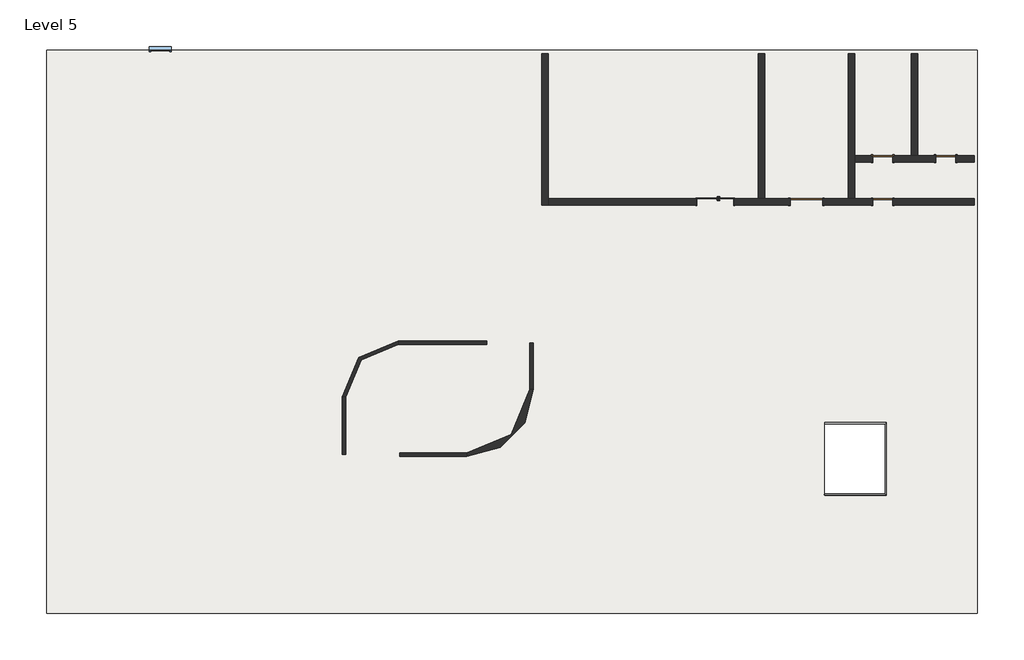
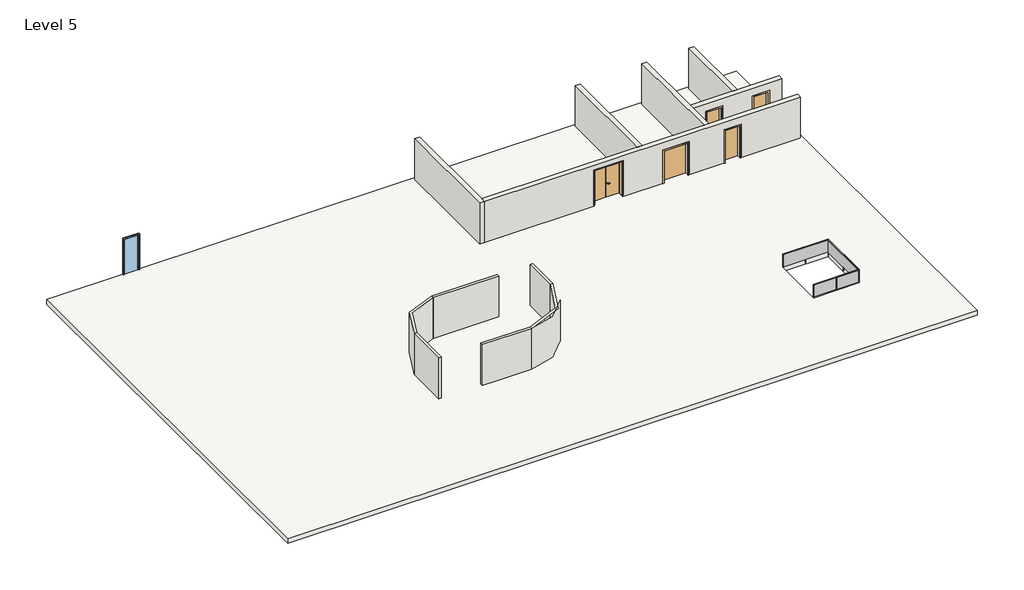
# One storey: 12 walls, 5 doors, 1 railing, 1 slab, 1 window.
"""IFC4 building model written with IfcOpenShell, lengths in millimetres."""

import ifcopenshell
import ifcopenshell.guid

model = None  # the IFC model being written
_history = None  # IfcOwnerHistory: only IFC2X3 demands one
_inside = {}  # id of a spatial element -> (the spatial element, [elements in it])
_under = {}  # id of a project, library or spatial element -> (it, [spatial elements below it])
_declared = {}  # id of a project -> (the project, [libraries it declares])
_typed = {}  # id of a type object -> (the type object, [elements of that type])
_made_of = {}  # id of a material, layer set ... -> (it, [elements and type objects made of it])


def new_model(schema):
    """Start an empty IFC model of exactly this schema.

    Asked for "IFC4X3", IfcOpenShell would pick the latest addendum, in which some entities
    have other attributes; the version numbers below select the first issue.
    IFC2X3 requires an IfcOwnerHistory on every rooted entity: one is made here for all.
    """
    global model, _history
    if schema == "IFC4X3":
        model = ifcopenshell.file(schema_version=(4, 3, 0, 0))
    else:
        model = ifcopenshell.file(schema=schema)
    _inside.clear()
    _under.clear()
    _declared.clear()
    _typed.clear()
    _made_of.clear()
    _history = None
    if model.schema == "IFC2X3":
        org = make("IfcOrganization", Name="unknown")
        user = make(
            "IfcPersonAndOrganization",
            ThePerson=make("IfcPerson", FamilyName="unknown"),
            TheOrganization=org,
        )
        app = make(
            "IfcApplication",
            ApplicationDeveloper=org,
            Version="unknown",
            ApplicationFullName="unknown",
            ApplicationIdentifier="unknown",
        )
        _history = make(
            "IfcOwnerHistory",
            OwningUser=user,
            OwningApplication=app,
            ChangeAction="ADDED",
            CreationDate=0,
        )
    return model


def make(cls, **values):
    """One entity of the class cls with the attributes given. An attribute that is None is left unset."""
    return model.create_entity(
        cls, **{name: value for name, value in values.items() if value is not None}
    )


def rooted(cls, **values):
    """An entity with a GlobalId (a new one), such as an element, a storey or a relation."""
    return make(cls, GlobalId=ifcopenshell.guid.new(), OwnerHistory=_history, **values)


def si_unit(unit_type, name, prefix=None):
    """IfcSIUnit, for example si_unit("LENGTHUNIT", "METRE", prefix="MILLI")."""
    return make("IfcSIUnit", UnitType=unit_type, Prefix=prefix, Name=name)


def assignment(units):
    """IfcUnitAssignment: the units of a project."""
    return None if units is None else make("IfcUnitAssignment", Units=units)


def point(xyz):
    """IfcCartesianPoint."""
    return None if xyz is None else make("IfcCartesianPoint", Coordinates=xyz)


def direction(xyz):
    """IfcDirection."""
    return None if xyz is None else make("IfcDirection", DirectionRatios=xyz)


def frame(location, z_axis=None, x_axis=None):
    """IfcAxis2Placement3D, a coordinate frame: its origin and axes. An axis left out is left unset."""
    return make(
        "IfcAxis2Placement3D",
        Location=point(location),
        Axis=direction(z_axis),
        RefDirection=direction(x_axis),
    )


def frame_2d(location, x_axis=None):
    """IfcAxis2Placement2D, a coordinate frame in the plane: its origin and x axis."""
    return make(
        "IfcAxis2Placement2D", Location=point(location), RefDirection=direction(x_axis)
    )


def origin():
    """The frame at (0, 0, 0) with its axes left unset."""
    return frame((0.0, 0.0, 0.0))


def origin_with_axes():
    """The frame at (0, 0, 0) with the z axis (0, 0, 1) and the x axis (1, 0, 0) written out."""
    return frame((0.0, 0.0, 0.0), z_axis=(0.0, 0.0, 1.0), x_axis=(1.0, 0.0, 0.0))


def place(relative_to, where):
    """IfcLocalPlacement: puts the frame where relative to a parent placement (None: the world)."""
    return make(
        "IfcLocalPlacement", PlacementRelTo=relative_to, RelativePlacement=where
    )


def context(
    kind, dimensions, precision=None, world=None, true_north=None, identifier=None
):
    """IfcGeometricRepresentationContext, for example the 3D "Model" context."""
    return make(
        "IfcGeometricRepresentationContext",
        ContextIdentifier=identifier,
        ContextType=kind,
        CoordinateSpaceDimension=dimensions,
        Precision=precision,
        WorldCoordinateSystem=world,
        TrueNorth=true_north,
    )


def project(units=None, contexts=None):
    """IfcProject with its units and contexts."""
    return rooted(
        "IfcProject",
        Name="project",
        RepresentationContexts=contexts,
        UnitsInContext=assignment(units),
    )


def spatial(cls, under=None, at=None, **own):
    """A site, building, storey or space (cls), placed at a placement, below another one or the project."""
    s = rooted(cls, ObjectPlacement=at, **own)
    if under is not None:
        _under.setdefault(under.id(), (under, []))[1].append(s)
    return s


def polyline(points):
    """IfcPolyline through the points."""
    return make("IfcPolyline", Points=[point(p) for p in points])


def circle_curve(where, radius):
    """IfcCircle in the frame where."""
    return make("IfcCircle", Position=where, Radius=radius)


def ellipse_curve(where, semi_axis1, semi_axis2):
    """IfcEllipse in the frame where."""
    return make(
        "IfcEllipse", Position=where, SemiAxis1=semi_axis1, SemiAxis2=semi_axis2
    )


def trimmed(basis, trim1, trim2, sense, master):
    """IfcTrimmedCurve: the piece of a basis curve between two trims."""
    return make(
        "IfcTrimmedCurve",
        BasisCurve=basis,
        Trim1=trim1,
        Trim2=trim2,
        SenseAgreement=sense,
        MasterRepresentation=master,
    )


def segment(curve, same_sense, transition):
    """IfcCompositeCurveSegment."""
    return make(
        "IfcCompositeCurveSegment",
        Transition=transition,
        SameSense=same_sense,
        ParentCurve=curve,
    )


def composite_curve(segments, self_intersect=None):
    """IfcCompositeCurve: segments joined end to end."""
    return make("IfcCompositeCurve", Segments=segments, SelfIntersect=self_intersect)


def outline(outer, holes=None, kind="AREA"):
    """IfcArbitraryClosedProfileDef: a profile drawn as a closed curve; with holes, ...WithVoids."""
    if holes is None:
        return make("IfcArbitraryClosedProfileDef", ProfileType=kind, OuterCurve=outer)
    return make(
        "IfcArbitraryProfileDefWithVoids",
        ProfileType=kind,
        OuterCurve=outer,
        InnerCurves=holes,
    )


def extrude(swept, where, along, depth):
    """IfcExtrudedAreaSolid: the profile swept, set in the frame where, extruded along a direction by depth."""
    return make(
        "IfcExtrudedAreaSolid",
        SweptArea=swept,
        Position=where,
        ExtrudedDirection=direction(along),
        Depth=depth,
    )


def faces_of(points, faces, orient=None, outer=None):
    """IfcFace entities. A face is a list of loops; a loop is a list of indices into points, from 0.

    orient and outer hold one flag for each loop. By default every Orientation is true, the
    first loop of a face is its IfcFaceOuterBound and the others are IfcFaceBound.
    """
    made = []
    for i, loops in enumerate(faces):
        bounds = []
        for j, loop in enumerate(loops):
            is_outer = j == 0 if outer is None else outer[i][j]
            bounds.append(
                make(
                    "IfcFaceOuterBound" if is_outer else "IfcFaceBound",
                    Bound=make("IfcPolyLoop", Polygon=[points[k] for k in loop]),
                    Orientation=True if orient is None else orient[i][j],
                )
            )
        made.append(make("IfcFace", Bounds=bounds))
    return made


def faceted_brep(points, faces, orient=None, outer=None, voids=None):
    """IfcFacetedBrep: a solid bounded by flat faces; with voids (closed shells), ...WithVoids."""
    shared = [point(p) for p in points]
    hull = make("IfcClosedShell", CfsFaces=faces_of(shared, faces, orient, outer))
    if voids is None:
        return make("IfcFacetedBrep", Outer=hull)
    return make(
        "IfcFacetedBrepWithVoids",
        Outer=hull,
        Voids=[
            make(cls, CfsFaces=faces_of(shared, fs, o, b)) for cls, fs, o, b in voids
        ],
    )


def shape(context_of_items, identifier, shape_type, items):
    """IfcShapeRepresentation: the items that make up one representation, for example the "Body"."""
    return make(
        "IfcShapeRepresentation",
        ContextOfItems=context_of_items,
        RepresentationIdentifier=identifier,
        RepresentationType=shape_type,
        Items=items,
    )


def source(mapping_origin, context_of_items, identifier, shape_type, items):
    """IfcRepresentationMap: a shape defined once, which mapped items show again and again."""
    return make(
        "IfcRepresentationMap",
        MappingOrigin=mapping_origin,
        MappedRepresentation=shape(context_of_items, identifier, shape_type, items),
    )


def transform(
    local_origin,
    x_axis=None,
    y_axis=None,
    z_axis=None,
    scale=None,
    scale2=None,
    scale3=None,
    uniform=True,
):
    """IfcCartesianTransformationOperator3D, or its non-uniform kind. x_axis, y_axis, z_axis: its Axis1, 2, 3."""
    if uniform:
        return make(
            "IfcCartesianTransformationOperator3D",
            Axis1=direction(x_axis),
            Axis2=direction(y_axis),
            LocalOrigin=point(local_origin),
            Scale=scale,
            Axis3=direction(z_axis),
        )
    return make(
        "IfcCartesianTransformationOperator3DnonUniform",
        Axis1=direction(x_axis),
        Axis2=direction(y_axis),
        LocalOrigin=point(local_origin),
        Scale=scale,
        Axis3=direction(z_axis),
        Scale2=scale2,
        Scale3=scale3,
    )


def mapped(mapping_source, mapping_target):
    """IfcMappedItem: shows the shape of a source again, moved by a transform."""
    return make(
        "IfcMappedItem", MappingSource=mapping_source, MappingTarget=mapping_target
    )


def made_of(thing, what):
    """Note that an element or type object is made of a material, layer set ...; save() writes the relation."""
    if what is not None:
        _made_of.setdefault(what.id(), (what, []))[1].append(thing)
    return thing


def element(
    cls,
    number,
    at=None,
    inside=None,
    cuts=None,
    type_object=None,
    material=None,
    context=None,
    identifier="Body",
    shape_type=None,
    held_by="IfcProductDefinitionShape",
    body=None,
    shapes=None,
    **own,
):
    """One element of the class cls, such as IfcWall. Its Tag is "e" and its number.

    at: its placement. inside: the storey or other place that contains it. cuts: it is an
    opening in that element (IfcRelVoidsElement). A single representation is given by context,
    identifier, shape_type and body (its items); several are given by shapes. held_by: the class
    of the entity that holds the representations. save() writes the other relations.
    """
    e = rooted(cls, Tag="e%d" % number, ObjectPlacement=at, **own)
    if body is not None:
        shapes = [shape(context, identifier, shape_type, body)]
    if shapes is not None:
        e.Representation = make(held_by, Representations=shapes)
    if inside is not None:
        _inside.setdefault(inside.id(), (inside, []))[1].append(e)
    if cuts is not None:
        rooted(
            "IfcRelVoidsElement", RelatingBuildingElement=cuts, RelatedOpeningElement=e
        )
    if type_object is not None:
        _typed.setdefault(type_object.id(), (type_object, []))[1].append(e)
    return made_of(e, material)


def aggregate(whole, parts):
    """IfcRelAggregates: a whole, such as a stair, and the parts it consists of."""
    return rooted("IfcRelAggregates", RelatingObject=whole, RelatedObjects=parts)


def save(model, path):
    """Write the relations noted so far, then the file.

    IfcRelAggregates (storeys below a building ...), IfcRelContainedInSpatialStructure (elements
    in a storey), IfcRelDefinesByType, IfcRelAssociatesMaterial and IfcRelDeclares: one each for
    every whole, place, type object, material and project.
    """
    for whole, parts in _under.values():
        aggregate(whole, parts)
    for where, things in _inside.values():
        rooted(
            "IfcRelContainedInSpatialStructure",
            RelatedElements=things,
            RelatingStructure=where,
        )
    for kind, things in _typed.values():
        rooted("IfcRelDefinesByType", RelatedObjects=things, RelatingType=kind)
    for what, things in _made_of.values():
        rooted("IfcRelAssociatesMaterial", RelatedObjects=things, RelatingMaterial=what)
    for by, libraries in _declared.values():
        rooted("IfcRelDeclares", RelatingContext=by, RelatedDefinitions=libraries)
    model.write(path)


def plane_surface(at):
    """IfcPlane: the flat surface through the origin of the frame at, square to its z axis."""
    return make("IfcPlane", Position=at)


def cylinder_surface(at, radius):
    """IfcCylindricalSurface: all points at the distance radius from the z axis of the frame at."""
    return make("IfcCylindricalSurface", Position=at, Radius=radius)


def advanced_brep(points, edges, surfaces, faces):
    """IfcAdvancedBrep: a solid bounded by faces that lie on surfaces and meet in shared edges.

    An edge is (start, end): straight between two places in points (the first is 0);
    or (start, end, curve); or (start, end, curve, False) where it runs against its curve.
    A face is (place in surfaces, loops), or (place, loops, False) where it looks against
    its surface's normal. A loop lists edges by number (the first is 1), with a minus sign
    where the edge is run from its end to its start. The first loop is the outer one.
    """
    corners = [point(p) for p in points]
    vertices = [make("IfcVertexPoint", VertexGeometry=c) for c in corners]
    made = []
    for start, end, *more in edges:
        made.append(
            make(
                "IfcEdgeCurve",
                EdgeStart=vertices[start],
                EdgeEnd=vertices[end],
                EdgeGeometry=more[0] if more else make("IfcPolyline", Points=[corners[start], corners[end]]),
                SameSense=more[1] if len(more) > 1 else True,
            )
        )
    hull = []
    for where, loops, *sense in faces:
        bounds = []
        for j, loop in enumerate(loops):
            ring = [make("IfcOrientedEdge", EdgeElement=made[abs(k) - 1], Orientation=k > 0) for k in loop]
            bounds.append(
                make(
                    "IfcFaceOuterBound" if j == 0 else "IfcFaceBound",
                    Bound=make("IfcEdgeLoop", EdgeList=ring),
                    Orientation=True,
                )
            )
        hull.append(make("IfcAdvancedFace", Bounds=bounds, FaceSurface=surfaces[where], SameSense=sense[0] if sense else True))
    return make("IfcAdvancedBrep", Outer=make("IfcClosedShell", CfsFaces=hull))


def door_double_flush_variable_door_double_flush_variable_ac6c3b87(model_context):
    return source(origin(), model_context, "Body", "SolidModel", [
        advanced_brep(
        [(90.0, 139.4346141, 1000.0), (110.0, 139.4346141, 1000.0), (90.0, 69.4346141, 1000.0), (110.0, 89.4346141, 1000.0), (220.0, 69.4346141, 1000.0), (220.0, 89.4346141, 1000.0)],
        [
            (0, 1, circle_curve(frame((100.0, 139.4346141, 1000.0), z_axis=(0.0, 1.0, 0.0), x_axis=(1.0, 0.0, 0.0)), 10.0)),
            (1, 0, circle_curve(frame((100.0, 139.4346141, 1000.0), z_axis=(0.0, 1.0, 0.0), x_axis=(1.0, 0.0, 0.0)), 10.0)),
            (0, 2),
            (2, 3, ellipse_curve(frame((100.0, 79.4346141, 1000.0), z_axis=(-0.7071067811865385, 0.7071067811865565, 0.0), x_axis=(0.7071067811865563, 0.7071067811865386, 0.0)), 14.1421356, 10.0)),
            (3, 1),
            (3, 2, ellipse_curve(frame((100.0, 79.4346141, 1000.0), z_axis=(-0.7071067811865385, 0.7071067811865565, 0.0), x_axis=(0.7071067811865563, 0.7071067811865386, 0.0)), 14.1421356, 10.0)),
            (4, 5, circle_curve(frame((220.0, 79.4346141, 1000.0), z_axis=(1.0, 0.0, 0.0), x_axis=(0.0, 1.0, 0.0)), 10.0)),
            (5, 4, circle_curve(frame((220.0, 79.4346141, 1000.0), z_axis=(1.0, 0.0, 0.0), x_axis=(0.0, 1.0, 0.0)), 10.0)),
            (2, 4),
            (5, 3),
        ],
        [
            plane_surface(frame((100.0, 139.4346141, -287.7526403), z_axis=(0.0, 1.0, 0.0), x_axis=(0.0, 0.0, 1.0))),
            cylinder_surface(frame((100.0, 139.4346141, 1000.0), z_axis=(0.0, 1.0, 0.0), x_axis=(1.0, 0.0, 0.0)), 10.0),
            plane_surface(frame((220.0, 79.4346141, -287.7526403), z_axis=(1.0, 0.0, 0.0), x_axis=(0.0, 0.0, 1.0))),
            cylinder_surface(frame((100.0, 79.4346141, 1000.0), z_axis=(-1.0, 0.0, 0.0), x_axis=(0.0, 1.0, 0.0)), 10.0),
        ],
        [
            (0, [[1, 2]]),
            (1, [[-1, 3, 4, 5]]),
            (1, [[-2, -5, 6, -3]]),
            (2, [[7, 8]]),
            (3, [[-4, 9, -8, 10]]),
            (3, [[-6, -10, -7, -9]]),
        ],
    ),
        advanced_brep(
        [(110.0, 199.4346141, 1000.0), (90.0, 199.4346141, 1000.0), (110.0, 229.4346141, 1000.0), (90.0, 249.4346141, 1000.0), (220.0, 229.4346141, 1000.0), (220.0, 249.4346141, 1000.0)],
        [
            (0, 1, circle_curve(frame((100.0, 199.4346141, 1000.0), z_axis=(0.0, -1.0, 0.0), x_axis=(-1.0, 0.0, 0.0)), 10.0)),
            (1, 0, circle_curve(frame((100.0, 199.4346141, 1000.0), z_axis=(0.0, -1.0, 0.0), x_axis=(-1.0, 0.0, 0.0)), 10.0)),
            (0, 2),
            (2, 3, ellipse_curve(frame((100.0, 239.4346141, 1000.0), z_axis=(-0.7071067811865475, -0.7071067811865475, 0.0), x_axis=(0.7071067811865474, -0.7071067811865476, 0.0)), 14.1421356, 10.0)),
            (3, 1),
            (3, 2, ellipse_curve(frame((100.0, 239.4346141, 1000.0), z_axis=(-0.7071067811865475, -0.7071067811865475, 0.0), x_axis=(0.7071067811865474, -0.7071067811865476, 0.0)), 14.1421356, 10.0)),
            (4, 5, circle_curve(frame((220.0, 239.4346141, 1000.0), z_axis=(1.0, 0.0, 0.0), x_axis=(0.0, 1.0, 0.0)), 10.0)),
            (5, 4, circle_curve(frame((220.0, 239.4346141, 1000.0), z_axis=(1.0, 0.0, 0.0), x_axis=(0.0, 1.0, 0.0)), 10.0)),
            (2, 4),
            (5, 3),
        ],
        [
            plane_surface(frame((100.0, 199.4346141, -287.7526403), z_axis=(0.0, -1.0, 0.0), x_axis=(0.0, 0.0, 1.0))),
            cylinder_surface(frame((100.0, 199.4346141, 1000.0), z_axis=(0.0, -1.0, 0.0), x_axis=(-1.0, 0.0, 0.0)), 10.0),
            plane_surface(frame((220.0, 239.4346141, -287.7526403), z_axis=(1.0, 0.0, 0.0), x_axis=(0.0, 0.0, 1.0))),
            cylinder_surface(frame((100.0, 239.4346141, 1000.0), z_axis=(-1.0, 0.0, 0.0), x_axis=(0.0, 1.0, 0.0)), 10.0),
        ],
        [
            (0, [[1, 2]]),
            (1, [[-1, 3, 4, 5]]),
            (1, [[-2, -5, 6, -3]]),
            (2, [[7, 8]]),
            (3, [[-4, 9, -8, 10]]),
            (3, [[-6, -10, -7, -9]]),
        ],
    ),
        extrude(outline(composite_curve([segment(trimmed(circle_curve(frame_2d((1000.0, 100.0)), 20.0), [point((1000.0, 80.0))], [point((1000.0, 120.0))], False, "CARTESIAN"), True, "CONTINUOUS"), segment(trimmed(circle_curve(frame_2d((1000.0, 100.0)), 20.0), [point((1000.0, 120.0))], [point((1000.0, 80.0))], False, "CARTESIAN"), True, "CONTINUOUS")], self_intersect=False)), frame((0.0, 129.4346141, 0.0), z_axis=(0.0, 1.0, 0.0), x_axis=(0.0, 0.0, 1.0)), (0.0, 0.0, 1.0), 10.0),
        extrude(outline(composite_curve([segment(trimmed(circle_curve(frame_2d((1000.0, 100.0)), 20.0), [point((1000.0, 80.0))], [point((1000.0, 120.0))], False, "CARTESIAN"), True, "CONTINUOUS"), segment(trimmed(circle_curve(frame_2d((1000.0, 100.0)), 20.0), [point((1000.0, 120.0))], [point((1000.0, 80.0))], False, "CARTESIAN"), True, "CONTINUOUS")], self_intersect=False)), frame((0.0, 189.4346141, 0.0), z_axis=(0.0, 1.0, 0.0), x_axis=(0.0, 0.0, 1.0)), (0.0, 0.0, 1.0), 10.0),
        extrude(outline(polyline([(0.0, 164.4346141), (-871.25, 164.4346141), (-871.25, 189.4346141), (0.0, 189.4346141), (0.0, 164.4346141)])), frame((0.0, 0.0, 100.0), z_axis=(0.0, 0.0, 1.0), x_axis=(1.0, 0.0, 0.0)), (0.0, 0.0, 1.0), 2250.0),
        extrude(outline(polyline([(871.25, 164.4346141), (0.0, 164.4346141), (0.0, 189.4346141), (871.25, 189.4346141), (871.25, 164.4346141)])), frame((0.0, 0.0, 100.0), z_axis=(0.0, 0.0, 1.0), x_axis=(1.0, 0.0, 0.0)), (0.0, 0.0, 1.0), 2250.0),
        faceted_brep([(905.75, -150.5653859, 100.0), (856.25, -150.5653859, 100.0), (856.25, 164.4346141, 100.0), (871.25, 164.4346141, 100.0), (871.25, 189.4346141, 100.0), (905.75, 189.4346141, 100.0), (905.75, 164.4346141, 100.0), (900.75, 164.4346141, 100.0), (900.75, 184.4346141, 100.0), (876.25, 184.4346141, 100.0), (876.25, 159.4346141, 100.0), (861.25, 159.4346141, 100.0), (861.25, -145.5653859, 100.0), (900.75, -145.5653859, 100.0), (900.75, -135.5653859, 100.0), (905.75, -135.5653859, 100.0), (905.75, -150.5653859, 2384.5), (-905.75, -150.5653859, 2384.5), (-905.75, -150.5653859, 100.0), (-856.25, -150.5653859, 100.0), (-856.25, -150.5653859, 2335.0), (856.25, -150.5653859, 2335.0), (856.25, 164.4346141, 2335.0), (-856.25, 164.4346141, 2335.0), (-856.25, 164.4346141, 100.0), (-871.25, 164.4346141, 100.0), (-871.25, 164.4346141, 2350.0), (871.25, 164.4346141, 2350.0), (871.25, 189.4346141, 2350.0), (-871.25, 189.4346141, 2350.0), (-871.25, 189.4346141, 100.0), (-905.75, 189.4346141, 100.0), (-905.75, 189.4346141, 2384.5), (905.75, 189.4346141, 2384.5), (905.75, 164.4346141, 2384.5), (-905.75, 164.4346141, 2384.5), (-905.75, 164.4346141, 100.0), (-900.75, 164.4346141, 100.0), (-900.75, 164.4346141, 2379.5), (900.75, 164.4346141, 2379.5), (900.75, 184.4346141, 2379.5), (-900.75, 184.4346141, 2379.5), (-900.75, 184.4346141, 100.0), (-876.25, 184.4346141, 100.0), (-876.25, 184.4346141, 2355.0), (876.25, 184.4346141, 2355.0), (876.25, 159.4346141, 2355.0), (-876.25, 159.4346141, 2355.0), (-876.25, 159.4346141, 100.0), (-861.25, 159.4346141, 100.0), (-861.25, 159.4346141, 2340.0), (861.25, 159.4346141, 2340.0), (861.25, -145.5653859, 2340.0), (-861.25, -145.5653859, 2340.0), (-861.25, -145.5653859, 100.0), (-900.75, -145.5653859, 100.0), (-900.75, -145.5653859, 2379.5), (900.75, -145.5653859, 2379.5), (900.75, -135.5653859, 2379.5), (-900.75, -135.5653859, 2379.5), (-900.75, -135.5653859, 100.0), (-905.75, -135.5653859, 100.0), (-905.75, -135.5653859, 2384.5), (905.75, -135.5653859, 2384.5)], [[[0, 1, 2, 3, 4, 5, 6, 7, 8, 9, 10, 11, 12, 13, 14, 15]], [[1, 0, 16, 17, 18, 19, 20, 21]], [[2, 1, 21, 22]], [[3, 2, 22, 23, 24, 25, 26, 27]], [[4, 3, 27, 28]], [[5, 4, 28, 29, 30, 31, 32, 33]], [[6, 5, 33, 34]], [[7, 6, 34, 35, 36, 37, 38, 39]], [[8, 7, 39, 40]], [[9, 8, 40, 41, 42, 43, 44, 45]], [[10, 9, 45, 46]], [[11, 10, 46, 47, 48, 49, 50, 51]], [[12, 11, 51, 52]], [[13, 12, 52, 53, 54, 55, 56, 57]], [[14, 13, 57, 58]], [[15, 14, 58, 59, 60, 61, 62, 63]], [[0, 15, 63, 16]], [[17, 62, 61, 18]], [[18, 61, 60, 55, 54, 49, 48, 43, 42, 37, 36, 31, 30, 25, 24, 19]], [[23, 20, 19, 24]], [[29, 26, 25, 30]], [[35, 32, 31, 36]], [[41, 38, 37, 42]], [[47, 44, 43, 48]], [[53, 50, 49, 54]], [[59, 56, 55, 60]], [[22, 21, 20, 23]], [[28, 27, 26, 29]], [[34, 33, 32, 35]], [[40, 39, 38, 41]], [[46, 45, 44, 47]], [[52, 51, 50, 53]], [[58, 57, 56, 59]], [[16, 63, 62, 17]]]),
    ])


def m_single_flush_0915_x_2134mm_1c84716f(model_context):
    return source(origin(), model_context, "Body", "SweptSolid", [
        extrude(outline(polyline([(2210.0, -533.5), (0.0, -533.5), (0.0, -457.5), (2134.0, -457.5), (2134.0, 457.5), (0.0, 457.5), (0.0, 533.5), (2210.0, 533.5), (2210.0, -533.5)])), frame((0.0, -175.0, 0.0), z_axis=(0.0, 1.0, 0.0), x_axis=(0.0, 0.0, 1.0)), (0.0, 0.0, 1.0), 25.0),
        extrude(outline(polyline([(2210.0, 533.5), (2210.0, -533.5), (0.0, -533.5), (0.0, -457.5), (2134.0, -457.5), (2134.0, 457.5), (0.0, 457.5), (0.0, 533.5), (2210.0, 533.5)])), frame((0.0, 150.0, 0.0), z_axis=(0.0, 1.0, 0.0), x_axis=(0.0, 0.0, 1.0)), (0.0, 0.0, 1.0), 25.0),
        extrude(outline(polyline([(457.5, -99.0), (457.5, -150.0), (-457.5, -150.0), (-457.5, -99.0), (457.5, -99.0)])), origin_with_axes(), (0.0, 0.0, 1.0), 2134.0),
    ])


def m_single_flush_1500_x_2134mm_2_edebd810(model_context):
    return source(origin(), model_context, "Body", "SweptSolid", [
        extrude(outline(polyline([(2210.0, -826.0), (0.0, -826.0), (0.0, -750.0), (2134.0, -750.0), (2134.0, 750.0), (0.0, 750.0), (0.0, 826.0), (2210.0, 826.0), (2210.0, -826.0)])), frame((0.0, -175.0, 0.0), z_axis=(0.0, 1.0, 0.0), x_axis=(0.0, 0.0, 1.0)), (0.0, 0.0, 1.0), 25.0),
        extrude(outline(polyline([(2210.0, 826.0), (2210.0, -826.0), (0.0, -826.0), (0.0, -750.0), (2134.0, -750.0), (2134.0, 750.0), (0.0, 750.0), (0.0, 826.0), (2210.0, 826.0)])), frame((0.0, 150.0, 0.0), z_axis=(0.0, 1.0, 0.0), x_axis=(0.0, 0.0, 1.0)), (0.0, 0.0, 1.0), 25.0),
        extrude(outline(polyline([(750.0, -99.0), (750.0, -150.0), (-750.0, -150.0), (-750.0, -99.0), (750.0, -99.0)])), origin_with_axes(), (0.0, 0.0, 1.0), 2134.0),
    ])


def glas_mpk_ffa405cb(model_context):
    return source(origin(), model_context, "Body", "SolidModel", [
        faceted_brep([(29194.1667192, -1196.642277, 12843.2628643), (29194.1667192, -1246.642277, 12843.2628643), (29194.1667192, -1246.642277, 12856.7371357), (29194.1667192, -1196.642277, 12856.7371357), (32034.1667192, -1196.642277, 12843.2628643), (31984.1667192, -1246.642277, 12843.2628643), (31984.1667192, -1246.642277, 12856.7371357), (32034.1667192, -1196.642277, 12856.7371357), (32034.1667192, -4537.3716232, 12843.2628643), (31984.1667192, -4487.3716232, 12843.2628643), (31984.1667192, -4487.3716232, 12856.7371357), (32034.1667192, -4537.3716232, 12856.7371357), (29194.1667192, -4537.3716232, 12843.2628643), (29194.1667192, -4537.3716232, 12856.7371357), (29194.1667192, -4487.3716232, 12856.7371357), (29194.1667192, -4487.3716232, 12843.2628643)], [[[0, 1, 2, 3]], [[1, 0, 4, 5]], [[2, 1, 5, 6]], [[3, 2, 6, 7]], [[0, 3, 7, 4]], [[5, 4, 8, 9]], [[6, 5, 9, 10]], [[7, 6, 10, 11]], [[4, 7, 11, 8]], [[12, 13, 14, 15]], [[9, 8, 12, 15]], [[10, 9, 15, 14]], [[11, 10, 14, 13]], [[8, 11, 13, 12]]]),
        faceted_brep([(29194.1667192, -1236.642277, 12842.8769824), (29194.1667192, -1222.4501531, 12842.8769824), (29194.1667192, -1222.4501531, 12042.8769824), (29194.1667192, -1236.642277, 12042.8769824), (31994.1667192, -1236.642277, 12842.8769824), (32008.3588432, -1222.4501531, 12842.8769824), (32008.3588432, -1222.4501531, 12042.8769824), (31994.1667192, -1236.642277, 12042.8769824), (31994.1667192, -4497.3716232, 12842.8769824), (32008.3588432, -4511.5637472, 12842.8769824), (32008.3588432, -4511.5637472, 12042.8769824), (31994.1667192, -4497.3716232, 12042.8769824), (29194.1667192, -4497.3716232, 12842.8769824), (29194.1667192, -4497.3716232, 12042.8769824), (29194.1667192, -4511.5637472, 12042.8769824), (29194.1667192, -4511.5637472, 12842.8769824)], [[[0, 1, 2, 3]], [[1, 0, 4, 5]], [[2, 1, 5, 6]], [[3, 2, 6, 7]], [[0, 3, 7, 4]], [[5, 4, 8, 9]], [[6, 5, 9, 10]], [[7, 6, 10, 11]], [[4, 7, 11, 8]], [[12, 13, 14, 15]], [[9, 8, 12, 15]], [[10, 9, 15, 14]], [[11, 10, 14, 13]], [[8, 11, 13, 12]]]),
        extrude(outline(polyline([(30625.4167192, -4512.3716232), (30625.4167192, -4537.3716232), (30600.4167192, -4537.3716232), (30600.4167192, -4512.3716232), (30625.4167192, -4512.3716232)])), frame((0.0, 0.0, 11800.0), z_axis=(0.0, 0.0, 1.0), x_axis=(1.0, 0.0, 0.0)), (0.0, 0.0, 1.0), 1043.2628643),
        extrude(outline(polyline([(32009.1667192, -2854.5069501), (32034.1667192, -2854.5069501), (32034.1667192, -2879.5069501), (32009.1667192, -2879.5069501), (32009.1667192, -2854.5069501)])), frame((0.0, 0.0, 11800.0), z_axis=(0.0, 0.0, 1.0), x_axis=(1.0, 0.0, 0.0)), (0.0, 0.0, 1.0), 1043.2628643),
        extrude(outline(polyline([(30600.4167192, -1221.642277), (30600.4167192, -1196.642277), (30625.4167192, -1196.642277), (30625.4167192, -1221.642277), (30600.4167192, -1221.642277)])), frame((0.0, 0.0, 11800.0), z_axis=(0.0, 0.0, 1.0), x_axis=(1.0, 0.0, 0.0)), (0.0, 0.0, 1.0), 1043.2628643),
        extrude(outline(polyline([(32009.1667192, -4522.3716232), (32034.1667192, -4522.3716232), (32034.1667192, -4547.3716232), (32009.1667192, -4547.3716232), (32009.1667192, -4522.3716232)])), frame((0.0, 0.0, 11800.0), z_axis=(0.0, 0.0, 1.0), x_axis=(1.0, 0.0, 0.0)), (0.0, 0.0, 1.0), 1043.2628643),
        extrude(outline(polyline([(32019.1667192, -1221.642277), (32019.1667192, -1196.642277), (32044.1667192, -1196.642277), (32044.1667192, -1221.642277), (32019.1667192, -1221.642277)])), frame((0.0, 0.0, 11800.0), z_axis=(0.0, 0.0, 1.0), x_axis=(1.0, 0.0, 0.0)), (0.0, 0.0, 1.0), 1043.2628643),
        extrude(outline(polyline([(29206.6667192, -4512.3716232), (29206.6667192, -4537.3716232), (29181.6667192, -4537.3716232), (29181.6667192, -4512.3716232), (29206.6667192, -4512.3716232)])), frame((0.0, 0.0, 11800.0), z_axis=(0.0, 0.0, 1.0), x_axis=(1.0, 0.0, 0.0)), (0.0, 0.0, 1.0), 1043.2628643),
        extrude(outline(polyline([(29194.1667192, -1221.642277), (29194.1667192, -1196.642277), (29219.1667192, -1196.642277), (29219.1667192, -1221.642277), (29194.1667192, -1221.642277)])), frame((0.0, 0.0, 11800.0), z_axis=(0.0, 0.0, 1.0), x_axis=(1.0, 0.0, 0.0)), (0.0, 0.0, 1.0), 1043.2628643),
    ])


def window_variable_standard_7c8c74e5(model_context):
    return source(origin(), model_context, "Body", "SolidModel", [
        extrude(outline(polyline([(9000.0, 500.0), (9000.0, -500.0), (1000.0, -500.0), (1000.0, 500.0), (9000.0, 500.0)]), holes=[polyline([(8920.0, 440.0), (1080.0, 440.0), (1080.0, -440.0), (8920.0, -440.0), (8920.0, 440.0)])]), frame((0.0, 10.0, 0.0), z_axis=(0.0, 1.0, 0.0), x_axis=(0.0, 0.0, 1.0)), (0.0, 0.0, 1.0), 60.0),
        faceted_brep([(470.0, 10.0, 8950.0), (470.0, -20.0, 8950.0), (470.0, -20.0, 1050.0), (470.0, 10.0, 1050.0), (-470.0, -20.0, 8950.0), (-470.0, -20.0, 1050.0), (410.0, -20.0, 1110.0), (-410.0, -20.0, 1110.0), (-410.0, -20.0, 8890.0), (410.0, -20.0, 8890.0), (-470.0, 10.0, 1050.0), (-470.0, 10.0, 8950.0), (440.0, 10.0, 8920.0), (-440.0, 10.0, 8920.0), (-440.0, 10.0, 1080.0), (440.0, 10.0, 1080.0), (440.0, 40.0, 8920.0), (440.0, 40.0, 1080.0), (-440.0, 40.0, 1080.0), (-440.0, 40.0, 8920.0), (410.0, 40.0, 8890.0), (-410.0, 40.0, 8890.0), (-410.0, 40.0, 1110.0), (410.0, 40.0, 1110.0)], [[[0, 1, 2, 3]], [[1, 4, 5, 2], [6, 7, 8, 9]], [[3, 2, 5, 10]], [[3, 10, 11, 0], [12, 13, 14, 15]], [[16, 12, 15, 17]], [[17, 15, 14, 18]], [[17, 18, 19, 16], [20, 21, 22, 23]], [[9, 20, 23, 6]], [[6, 23, 22, 7]], [[10, 5, 4, 11]], [[18, 14, 13, 19]], [[7, 22, 21, 8]], [[11, 4, 1, 0]], [[19, 13, 12, 16]], [[8, 21, 20, 9]]]),
        extrude(outline(polyline([(-500.0, -180.0), (-500.0, 10.0), (500.0, 10.0), (500.0, -180.0), (-500.0, -180.0)])), frame((0.0, 0.0, 1005.0), z_axis=(0.0, 0.0, 1.0), x_axis=(1.0, 0.0, 0.0)), (0.0, 0.0, 1.0), 15.0),
        extrude(outline(polyline([(80.0221543, 1020.0), (180.0, 1000.0), (180.0, 990.0), (178.0, 990.0), (178.0, 998.3604634), (79.8240723, 1018.0), (70.0, 1018.0), (70.0, 1020.0), (80.0221543, 1020.0)])), frame((-500.0, 0.0, 0.0), z_axis=(1.0, 0.0, 0.0), x_axis=(0.0, 1.0, 0.0)), (0.0, 0.0, 1.0), 1000.0),
        extrude(outline(polyline([(410.0, -5.0), (-410.0, -5.0), (-410.0, 25.0), (410.0, 25.0), (410.0, -5.0)])), frame((0.0, 0.0, 1110.0), z_axis=(0.0, 0.0, 1.0), x_axis=(1.0, 0.0, 0.0)), (0.0, 0.0, 1.0), 7780.0),
    ])


model = new_model("IFC4")

# Units and contexts
model_context = context("Model", 3, world=origin())
ifc_project = project(units=[si_unit("LENGTHUNIT", "METRE", prefix="MILLI")], contexts=[model_context])

# Site, building, storey
site = spatial("IfcSite", under=ifc_project)
building = spatial("IfcBuilding", under=site)
storey = spatial("IfcBuildingStorey", under=building, Name="Level 5", Elevation=12000.0)

# Doors
placement = place(None, origin())
door_double_flush_variable_door_double_flush_variable_shape = door_double_flush_variable_door_double_flush_variable_ac6c3b87(model_context)
element("IfcDoor", 1, ObjectType="Door Double Flush - Variable : Door Double Flush - Variable", at=placement, inside=storey, context=model_context, shape_type="MappedRepresentation", body=[
    mapped(door_double_flush_variable_door_double_flush_variable_shape, transform((24136.7471367, 8984.3231089, 12000.0), x_axis=(1.0, 0.0, 0.0), y_axis=(0.0, 1.0, 0.0), z_axis=(0.0, 0.0, 1.0))),
])
m_single_flush_0915_x_2134mm_shape = m_single_flush_0915_x_2134mm_1c84716f(model_context)
element("IfcDoor", 2, ObjectType="M_Single-Flush : 0915 x 2134mm", at=placement, inside=storey, context=model_context, shape_type="MappedRepresentation", body=[
    mapped(m_single_flush_0915_x_2134mm_shape, transform((34787.1221367, 10998.757723, 12000.0), x_axis=(-1.0, 0.0, 0.0), y_axis=(0.0, -1.0, 0.0), z_axis=(0.0, 0.0, 1.0))),
])
element("IfcDoor", 3, ObjectType="M_Single-Flush : 0915 x 2134mm", at=placement, inside=storey, context=model_context, shape_type="MappedRepresentation", body=[
    mapped(m_single_flush_0915_x_2134mm_shape, transform((31874.3721367, 10998.757723, 12000.0), x_axis=(-1.0, 0.0, 0.0), y_axis=(0.0, -1.0, 0.0), z_axis=(0.0, 0.0, 1.0))),
])
element("IfcDoor", 4, ObjectType="M_Single-Flush : 0915 x 2134mm", at=placement, inside=storey, context=model_context, shape_type="MappedRepresentation", body=[
    mapped(m_single_flush_0915_x_2134mm_shape, transform((31874.3721367, 8998.757723, 12000.0), x_axis=(-1.0, 0.0, 0.0), y_axis=(0.0, -1.0, 0.0), z_axis=(0.0, 0.0, 1.0))),
])
m_single_flush_1500_x_2134mm_2_shape = m_single_flush_1500_x_2134mm_2_edebd810(model_context)
element("IfcDoor", 5, ObjectType="M_Single-Flush : 1500 x 2134mm 2", at=placement, inside=storey, context=model_context, shape_type="MappedRepresentation", body=[
    mapped(m_single_flush_1500_x_2134mm_2_shape, transform((28342.9971367, 8998.757723, 12000.0), x_axis=(-1.0, 0.0, 0.0), y_axis=(0.0, -1.0, 0.0), z_axis=(0.0, 0.0, 1.0))),
])

# Railing
glas_mpk_shape = glas_mpk_ffa405cb(model_context)
element("IfcRailing", 6, ObjectType="Glas - MPK", at=placement, inside=storey, context=model_context, shape_type="MappedRepresentation", body=[
    mapped(glas_mpk_shape, transform((0.0, 0.0, 0.0), x_axis=(1.0, 0.0, 0.0), y_axis=(0.0, 1.0, 0.0), z_axis=(0.0, 0.0, 1.0))),
])

# Slab
element("IfcSlab", 7, ObjectType="Generic 300mm", at=placement, inside=storey, context=model_context, shape_type="SweptSolid", body=[
    extrude(outline(polyline([(-6732.0028633, 15998.757723), (36243.4971367, 15998.757723), (36243.4971367, -10001.242277), (-6732.0028633, -10001.242277), (-6732.0028633, 15998.757723)]), holes=[polyline([(32044.1667192, -1186.642277), (29194.1667192, -1186.642277), (29194.1667192, -4547.3716232), (32044.1667192, -4547.3716232), (32044.1667192, -1186.642277)])]), frame((0.0, 0.0, 11700.0), z_axis=(0.0, 0.0, 1.0), x_axis=(1.0, 0.0, 0.0)), (0.0, 0.0, 1.0), 300.0),
])

# Walls
element("IfcWall", 8, ObjectType="Generic - 300mm", at=placement, inside=storey, context=model_context, shape_type="Brep", body=[
    faceted_brep([(16117.9971367, 15848.757723, 12000.0), (16117.9971367, 8848.757723, 12000.0), (16117.9971367, 8848.757723, 14700.0), (16117.9971367, 15848.757723, 14700.0), (16417.9971367, 15848.757723, 12000.0), (16417.9971367, 15848.757723, 14700.0), (16417.9971367, 9148.757723, 14700.0), (16417.9971367, 8848.757723, 14700.0), (16417.9971367, 8848.757723, 12000.0), (16417.9971367, 9148.757723, 12000.0)], [[[0, 1, 2, 3]], [[4, 5, 6, 7, 8, 9]], [[1, 0, 4, 9, 8]], [[3, 2, 7, 6, 5]], [[2, 1, 8, 7]], [[0, 3, 5, 4]]]),
])
element("IfcWall", 9, ObjectType="Generic - 300mm", at=placement, inside=storey, context=model_context, shape_type="SweptSolid", body=[
    extrude(outline(polyline([(26117.9971367, 9148.757723), (26117.9971367, 15848.757723), (26417.9971367, 15848.757723), (26417.9971367, 9148.757723), (26117.9971367, 9148.757723)])), frame((0.0, 0.0, 12000.0), z_axis=(0.0, 0.0, 1.0), x_axis=(1.0, 0.0, 0.0)), (0.0, 0.0, 1.0), 2700.0),
])
element("IfcWall", 10, ObjectType="Generic - 300mm", at=placement, inside=storey, context=model_context, shape_type="Brep", body=[
    faceted_brep([(30267.9971367, 15848.757723, 12000.0), (30267.9971367, 9148.757723, 12000.0), (30267.9971367, 9148.757723, 14700.0), (30267.9971367, 15848.757723, 14700.0), (30567.9971367, 15848.757723, 12000.0), (30567.9971367, 15848.757723, 14700.0), (30567.9971367, 11148.757723, 14700.0), (30567.9971367, 10848.757723, 14700.0), (30567.9971367, 9148.757723, 14700.0), (30567.9971367, 9148.757723, 12000.0), (30567.9971367, 10848.757723, 12000.0), (30567.9971367, 11148.757723, 12000.0)], [[[0, 1, 2, 3]], [[4, 5, 6, 7, 8, 9, 10, 11]], [[1, 0, 4, 11, 10, 9]], [[3, 2, 8, 7, 6, 5]], [[2, 1, 9, 8]], [[0, 3, 5, 4]]]),
])
element("IfcWall", 11, ObjectType="Generic - 300mm", at=placement, inside=storey, context=model_context, shape_type="SweptSolid", body=[
    extrude(outline(polyline([(33180.7471367, 11148.757723), (33180.7471367, 15848.757723), (33480.7471367, 15848.757723), (33480.7471367, 11148.757723), (33180.7471367, 11148.757723)])), frame((0.0, 0.0, 12000.0), z_axis=(0.0, 0.0, 1.0), x_axis=(1.0, 0.0, 0.0)), (0.0, 0.0, 1.0), 2700.0),
])
element("IfcWall", 12, ObjectType="Generic - 300mm", at=placement, inside=storey, context=model_context, shape_type="Brep", body=[
    faceted_brep([(16417.9971367, 9148.757723, 14700.0), (26117.9971367, 9148.757723, 14700.0), (26417.9971367, 9148.757723, 14700.0), (30267.9971367, 9148.757723, 14700.0), (30567.9971367, 9148.757723, 14700.0), (36093.4971367, 9148.757723, 14700.0), (36093.4971367, 9148.757723, 12000.0), (32331.8721367, 9148.757723, 12000.0), (32331.8721367, 9148.757723, 14134.0), (31416.8721367, 9148.757723, 14134.0), (31416.8721367, 9148.757723, 12000.0), (30567.9971367, 9148.757723, 12000.0), (30267.9971367, 9148.757723, 12000.0), (29092.9971367, 9148.757723, 12000.0), (29092.9971367, 9148.757723, 14134.0), (27592.9971367, 9148.757723, 14134.0), (27592.9971367, 9148.757723, 12000.0), (26417.9971367, 9148.757723, 12000.0), (26117.9971367, 9148.757723, 12000.0), (25017.9971367, 9148.757723, 12000.0), (25017.9971367, 9148.757723, 14360.0), (23255.4971367, 9148.757723, 14360.0), (23255.4971367, 9148.757723, 12000.0), (16417.9971367, 9148.757723, 12000.0), (36093.4971367, 8848.757723, 14700.0), (16417.9971367, 8848.757723, 14700.0), (16417.9971367, 8848.757723, 12000.0), (23255.4971367, 8848.757723, 12000.0), (23255.4971367, 8848.757723, 14360.0), (25017.9971367, 8848.757723, 14360.0), (25017.9971367, 8848.757723, 12000.0), (27592.9971367, 8848.757723, 12000.0), (27592.9971367, 8848.757723, 14134.0), (29092.9971367, 8848.757723, 14134.0), (29092.9971367, 8848.757723, 12000.0), (31416.8721367, 8848.757723, 12000.0), (31416.8721367, 8848.757723, 14134.0), (32331.8721367, 8848.757723, 14134.0), (32331.8721367, 8848.757723, 12000.0), (36093.4971367, 8848.757723, 12000.0)], [[[0, 1, 2, 3, 4, 5, 6, 7, 8, 9, 10, 11, 12, 13, 14, 15, 16, 17, 18, 19, 20, 21, 22, 23]], [[24, 25, 26, 27, 28, 29, 30, 31, 32, 33, 34, 35, 36, 37, 38, 39]], [[26, 23, 22, 27]], [[10, 35, 34, 13, 12, 11]], [[38, 7, 6, 39]], [[16, 31, 30, 19, 18, 17]], [[5, 4, 3, 2, 1, 0, 25, 24]], [[0, 23, 26, 25]], [[36, 35, 10, 9]], [[37, 36, 9, 8]], [[38, 37, 8, 7]], [[32, 31, 16, 15]], [[33, 32, 15, 14]], [[34, 33, 14, 13]], [[29, 20, 19, 30]], [[20, 29, 28, 21]], [[21, 28, 27, 22]], [[6, 5, 24, 39]]]),
])
element("IfcWall", 13, ObjectType="Generic - 300mm", at=placement, inside=storey, context=model_context, shape_type="Brep", body=[
    faceted_brep([(31416.8721367, 11148.757723, 14134.0), (31416.8721367, 11148.757723, 12000.0), (30567.9971367, 11148.757723, 12000.0), (30567.9971367, 11148.757723, 14700.0), (33180.7471367, 11148.757723, 14700.0), (33480.7471367, 11148.757723, 14700.0), (36093.4971367, 11148.757723, 14700.0), (36093.4971367, 11148.757723, 12000.0), (35244.6221367, 11148.757723, 12000.0), (35244.6221367, 11148.757723, 14134.0), (34329.6221367, 11148.757723, 14134.0), (34329.6221367, 11148.757723, 12000.0), (33480.7471367, 11148.757723, 12000.0), (33180.7471367, 11148.757723, 12000.0), (32331.8721367, 11148.757723, 12000.0), (32331.8721367, 11148.757723, 14134.0), (30567.9971367, 10848.757723, 12000.0), (31416.8721367, 10848.757723, 12000.0), (31416.8721367, 10848.757723, 14134.0), (32331.8721367, 10848.757723, 14134.0), (32331.8721367, 10848.757723, 12000.0), (34329.6221367, 10848.757723, 12000.0), (34329.6221367, 10848.757723, 14134.0), (35244.6221367, 10848.757723, 14134.0), (35244.6221367, 10848.757723, 12000.0), (36093.4971367, 10848.757723, 12000.0), (36093.4971367, 10848.757723, 14700.0), (30567.9971367, 10848.757723, 14700.0)], [[[0, 1, 2, 3, 4, 5, 6, 7, 8, 9, 10, 11, 12, 13, 14, 15]], [[16, 17, 18, 19, 20, 21, 22, 23, 24, 25, 26, 27]], [[8, 7, 25, 24]], [[2, 1, 17, 16]], [[14, 13, 12, 11, 21, 20]], [[6, 5, 4, 3, 27, 26]], [[3, 2, 16, 27]], [[22, 21, 11, 10]], [[23, 22, 10, 9]], [[24, 23, 9, 8]], [[18, 17, 1, 0]], [[19, 18, 0, 15]], [[20, 19, 15, 14]], [[7, 6, 26, 25]]]),
])
element("IfcWall", 14, ObjectType="Interior - Blockwork 140", at=placement, inside=storey, context=model_context, shape_type="SweptSolid", body=[
    extrude(outline(polyline([(13583.5160614, 2407.0363043), (9501.5160614, 2407.0363043), (9501.5160614, 2571.0363043), (13583.5160614, 2571.0363043), (13583.5160614, 2407.0363043)])), frame((0.0, 0.0, 12000.0), z_axis=(0.0, 0.0, 1.0), x_axis=(1.0, 0.0, 0.0)), (0.0, 0.0, 1.0), 2700.0),
])
element("IfcWall", 15, ObjectType="Interior - Blockwork 140", at=placement, inside=storey, context=model_context, shape_type="SweptSolid", body=[
    extrude(outline(polyline([(7083.5160614, -10.9636957), (7083.5160614, -2674.9636957), (6919.5160614, -2674.9636957), (6919.5160614, -10.9636957), (7083.5160614, -10.9636957)])), frame((0.0, 0.0, 12000.0), z_axis=(0.0, 0.0, 1.0), x_axis=(1.0, 0.0, 0.0)), (0.0, 0.0, 1.0), 2700.0),
])
element("IfcWall", 16, ObjectType="Interior - Blockwork 140", at=placement, inside=storey, context=model_context, shape_type="SweptSolid", body=[
    extrude(outline(polyline([(9583.5160614, -2592.9636957), (12665.5160614, -2592.9636957), (12665.5160614, -2756.9636957), (9583.5160614, -2756.9636957), (9583.5160614, -2592.9636957)])), frame((0.0, 0.0, 12000.0), z_axis=(0.0, 0.0, 1.0), x_axis=(1.0, 0.0, 0.0)), (0.0, 0.0, 1.0), 2700.0),
])
element("IfcWall", 17, ObjectType="Interior - Blockwork 140", at=placement, inside=storey, context=model_context, shape_type="SweptSolid", body=[
    extrude(outline(polyline([(15583.5160614, 325.0363043), (15583.5160614, 2489.0363043), (15747.5160614, 2489.0363043), (15747.5160614, 325.0363043), (15583.5160614, 325.0363043)])), frame((0.0, 0.0, 12000.0), z_axis=(0.0, 0.0, 1.0), x_axis=(1.0, 0.0, 0.0)), (0.0, 0.0, 1.0), 2700.0),
])
element("IfcWall", 18, ObjectType="Interior - Blockwork 140", at=placement, inside=storey, context=model_context, shape_type="SweptSolid", body=[
    extrude(outline(composite_curve([segment(polyline([(7083.5160614, -10.9636957), (6919.5160614, -10.9636957)]), True, "CONTINUOUS"), segment(trimmed(circle_curve(frame_2d((9501.5160614, -10.9636957)), 2582.0), [point((6919.5160614, -10.9636957))], [point((9501.5160614, 2571.0363043))], False, "CARTESIAN"), True, "CONTINUOUS"), segment(polyline([(9501.5160614, 2571.0363043), (9501.5160614, 2407.0363043)]), True, "CONTINUOUS"), segment(trimmed(circle_curve(frame_2d((9501.5160614, -10.9636957)), 2418.0), [point((9501.5160614, 2407.0363043))], [point((7083.5160614, -10.9636957))], True, "CARTESIAN"), True, "CONTINUOUS")], self_intersect=False)), frame((0.0, 0.0, 12000.0), z_axis=(0.0, 0.0, 1.0), x_axis=(1.0, 0.0, 0.0)), (0.0, 0.0, 1.0), 2700.0),
])
element("IfcWall", 19, ObjectType="Interior - Blockwork 140", at=placement, inside=storey, context=model_context, shape_type="SweptSolid", body=[
    extrude(outline(composite_curve([segment(polyline([(15583.5160614, 325.0363043), (15747.5160614, 325.0363043)]), True, "CONTINUOUS"), segment(trimmed(circle_curve(frame_2d((12665.5160614, 325.0363043)), 3082.0), [point((15747.5160614, 325.0363043))], [point((12665.5160614, -2756.9636957))], False, "CARTESIAN"), True, "CONTINUOUS"), segment(polyline([(12665.5160614, -2756.9636957), (12665.5160614, -2592.9636957)]), True, "CONTINUOUS"), segment(trimmed(circle_curve(frame_2d((12665.5160614, 325.0363043)), 2918.0), [point((12665.5160614, -2592.9636957))], [point((15583.5160614, 325.0363043))], True, "CARTESIAN"), True, "CONTINUOUS")], self_intersect=False)), frame((0.0, 0.0, 12000.0), z_axis=(0.0, 0.0, 1.0), x_axis=(1.0, 0.0, 0.0)), (0.0, 0.0, 1.0), 2700.0),
])

# Window
window_variable_standard_shape = window_variable_standard_7c8c74e5(model_context)
element("IfcWindow", 20, ObjectType="Window - Variable : Standard", at=placement, inside=storey, context=model_context, shape_type="MappedRepresentation", body=[
    mapped(window_variable_standard_shape, transform((-1482.0028633, 15998.757723, 5400.0), x_axis=(-1.0, 0.0, 0.0), y_axis=(0.0, -1.0, 0.0), z_axis=(0.0, 0.0, 1.0))),
])

save(model, "model.ifc")

# Revit data of these elements
# Type "Door Double Flush - Variable : Door Double Flush - Variable"
#   Type Mark = "33"
#   Operation = "DoubleDoorSingleSwing"
#   Keynote = "16.03"
#   Rough Width [instance default] = 2.010 m
#   Rough Height [instance default] = 2.360 m
#   Doorhandle Height = 0.900 m
#   Height [instance default] = 2.260 m
#   Sill Height [instance default] = 0.100 m
#   Width [instance default] = 2.010 m
#   Visibility [instance default] = yes
#   Doorhandle choose [instance default] = element 138974
#   Doorhandle [instance default] = Metal _ Chrome
#   Door [instance default] = Door - Wood
#   Frame [instance default] = Door - Wood
#   Function = (empty or 0)
#   Wall Closure = (empty or 0)
#   Assembly Code = ""
# Type "M_Single-Flush : 0915 x 2134mm"
#   Type Mark = "20"
#   Thickness = 0.051 m
#   Height = 2.134 m
#   Trim Projection Ext = 0.025 m
#   Trim Projection Int = 0.025 m
#   Trim Width = 0.076 m
#   Width = 0.915 m
#   Door Material = Door - Panel
#   Frame Material = Door - Frame
#   Function = (empty or 0)
#   Wall Closure = (empty or 0)
# Type "M_Single-Flush : 1500 x 2134mm 2"
#   Type Mark = "34"
#   Thickness = 0.051 m
#   Height = 2.134 m
#   Trim Projection Ext = 0.025 m
#   Trim Projection Int = 0.025 m
#   Trim Width = 0.076 m
#   Width = 1.500 m
#   Door Material = Door - Panel
#   Frame Material = Door - Frame
#   Function = (empty or 0)
#   Wall Closure = (empty or 0)
# Type "Glas - MPK"
#   built-in parameter 1008619 = -0.0410105 (stored number, unit not read)
#   built-in parameter 1008612 = 0.019685 (stored number, unit not read)
#   built-in parameter 1008611 = 0.0984252 (stored number, unit not read)
#   built-in parameter 1008609 = 6.56168 (stored number, unit not read)
#   built-in parameter 1008604 = 0.19685 (stored number, unit not read)
#   built-in parameter 1008603 = 0.164042 (stored number, unit not read)
#   Railing Height = 0.865 m
#   built-in parameter 1008630 = 2
#   built-in parameter 1008610 = 1
#   built-in parameter 1008605 = 1
# Type "Generic 300mm"
#   Function = 0
#   Layers, outside or top first: 0.300 m no material (function 1)
# Type "Generic - 300mm"
#   Layers, outside or top first: 0.300 m no material (function 1)
# Type "Interior - Blockwork 140"
#   Layers, outside or top first: 0.012 m "Plasterboard" (function 5); 0.140 m "Masonry - Concrete Block" (function 1); 0.012 m "Plasterboard" (function 5)
# Type "Window - Variable : Standard"
#   Type Mark = "19"
#   Operation = "SinglePanel"
#   Keynote = "16.05.01"
#   Analytic Construction = "<None>"
#   Rough Width [instance default] = 1.010 m
#   Rough Height [instance default] = 1.010 m
#   Frame Depth = 0.060 m
#   Frame Height Bottom = 0.080 m
#   Frame Height Top = 0.080 m
#   Frame Width = 0.060 m
#   Height [instance default] = 1.010 m
#   Window Inset = 0.060 m
#   Window Width = 0.060 m
#   Instalation Depth [instance default] = 0.080 m
#   Width [instance default] = 1.010 m
#   Folding Wing [instance default] = no
#   Oppening Direction Vertical [instance default] = yes
#   Oppening Direction Visibility [instance default] = no
#   Casement [instance default] = yes
#   Frame [instance default] = none
#   Glas [instance default] = none
#   Window [instance default] = none
#   Windowsill Inside [instance default] = none
#   Windowsill Outside [instance default] = none
#   Wall Closure = (empty or 0)
#   Assembly Code = ""
# Element 1 (IfcDoor, "Door Double Flush - Variable : Door Double Flush - Variable")
#   Width = 1.7625 m
#   Sill Height = 0.100 m
#   Rough Width = 1.7625 m
#   Rough Height = 2.360 m
#   Height = 2.260 m
#   Visibility = yes
#   Frame = Door - Wood
#   Doorhandle choose = element 138974
#   Doorhandle = Metal _ Chrome
#   Door = Door - Wood
#   Phase Created = New Construction
#   Materials on its faces: "Door - Wood", "Metal _ Chrome"
# Elements 2, 3, 4 (IfcDoor, "M_Single-Flush : 0915 x 2134mm")
#   Phase Created = New Construction
#   Materials on its faces: "Door - Frame", "Door - Panel"
# Element 5 (IfcDoor, "M_Single-Flush : 1500 x 2134mm 2")
#   Phase Created = New Construction
#   Materials on its faces: "Door - Frame", "Door - Panel"
# Element 6 (IfcRailing, "Glas - MPK")
#   Phase Created = New Construction
#   Materials on its faces: "Metal - Aluminum", "Window - Glass"
# Element 7 (IfcSlab, "Generic 300mm")
#   built-in parameter 1001955 = 3.14159 (stored number, unit not read)
#   Height Offset From Level = 0.000 m
#   Phase Created = New Construction
#   Materials on its faces: "Default Floor"
# Elements 8, 9, 10, 11, 12, 13 (IfcWall, "Generic - 300mm")
#   Top Offset = -0.300 m
#   Base Offset = 0.000 m
#   wall height = 2.700 m
#   Phase Created = New Construction
#   Base Constraint = Level 5
#   Top Constraint = Level 6
#   Materials on its faces: "Default Wall"
# Elements 14, 15, 16, 17 (IfcWall, "Interior - Blockwork 140")
#   Top Offset = -0.300 m
#   Base Offset = 0.000 m
#   wall height = 2.700 m
#   Phase Created = New Construction
#   Base Constraint = Level 5
#   Top Constraint = Level 6
#   Materials on its faces: "Default Wall", "Plasterboard"
# Elements 18, 19 (IfcWall, "Interior - Blockwork 140")
#   Top Offset = -0.300 m
#   Base Offset = 0.000 m
#   Unconnected Height = 4.000 m
#   wall height = 2.700 m
#   Phase Created = New Construction
#   Materials on its faces: "Default Wall", "Plasterboard"
# Element 20 (IfcWindow, "Window - Variable : Standard")
#   Mark = "5"
#   Width = 1.000 m
#   Rough Width = 1.000 m
#   Rough Height = 8.000 m
#   Instalation Depth = 0.080 m
#   Height = 8.000 m
#   Oppening Direction Visibility = no
#   Oppening Direction Vertical = yes
#   Folding Wing = no
#   Casement = yes
#   Windowsill Outside = none
#   Windowsill Inside = none
#   Window = none
#   Glas = none
#   Frame = none
#   Phase Created = New Construction
#   Materials on its faces: "Plastic - White", "Metal _ Aluminium", "Wood - Birch", "Glass"
# Materials
#   "Metal _ Chrome": class "Metall", colour RGB 247 247 247, transparency 0
#   "Door - Wood": class "Unassigned", colour RGB 114 94 79, transparency 0
#   "Door - Panel": class "Wood", colour RGB 210 159 95, transparency 0
#   "Door - Frame": class "Miscellaneous", colour RGB 118 70 51, transparency 0
#   "Plasterboard": class "Drywall", colour RGB 249 249 249, transparency 0, Description = "Interior finish"
#   "Masonry - Concrete Block": class "Concrete", colour RGB 181 181 181, transparency 0
#   "Metal - Aluminum": class "Unassigned", colour RGB 247 247 247, transparency 0, Comments = "Rendering appearance not upgraded "
#   "Window - Glass": class "Glas", colour RGB 128 128 255, transparency 0.75
#   "Default Floor": class "Miscellaneous", colour RGB 127 127 127, transparency 0
#   "Default Wall": class "Miscellaneous", colour RGB 128 128 128, transparency 0
#   "Plastic - White": class "Kunststoff", colour RGB 249 249 249, transparency 0
#   "Metal _ Aluminium": class "Metall", colour RGB 247 247 247, transparency 0
#   "Wood - Birch": class "Holz", colour RGB 213 164 103, transparency 0
#   "Glass": class "Glass", colour RGB 0 128 192, transparency 0.9
